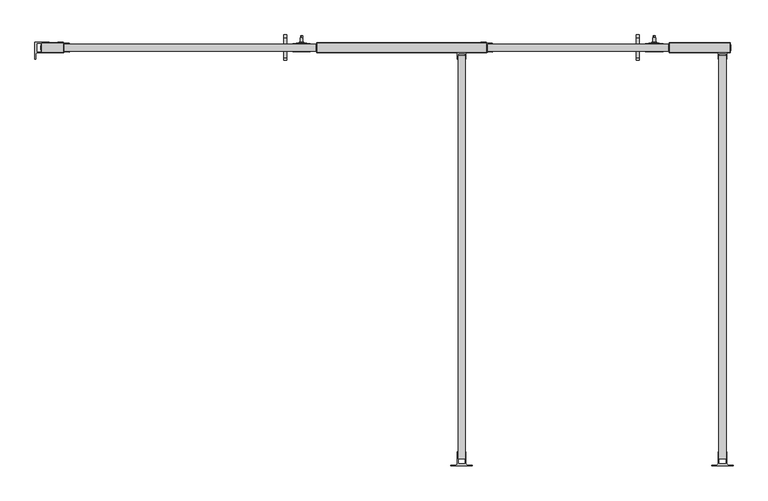
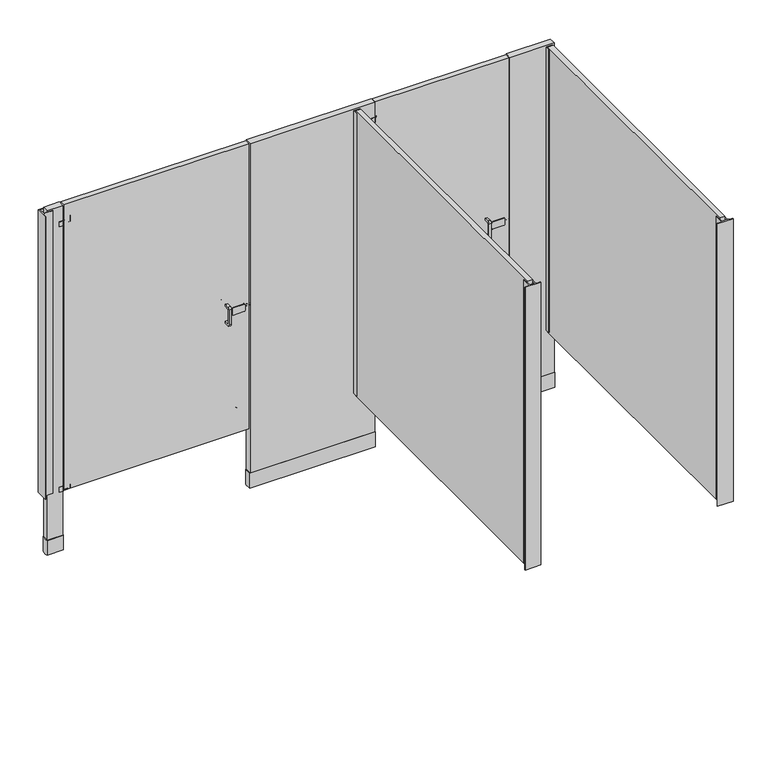
"""IFC4 building model written with IfcOpenShell, lengths in millimetres: proxy geometry, Partition-Floor_Braced-Bradley_Corp-St_Stl-ADA-N_Stalls : ADA (optional) + n Standard Stalls."""

from ifc_helpers import new_model, si_unit, point, frame, frame_2d, origin, origin_with_axes, place, context, project, spatial, polyline, circle_curve, ellipse_curve, trimmed, segment, composite_curve, outline, extrude, source, transform, mapped, element, save
from ifc_brep_helpers import plane_surface, cylinder_surface, revolved_surface, advanced_brep


def specialty_equipment_70690a28(model_context):
    return source(origin(), model_context, "Body", "SolidModel", [
        extrude(outline(composite_curve([segment(polyline([(1469.3891724, 988.06), (1492.2491724, 988.06), (1492.2491724, 977.9), (1469.3891724, 977.9)]), True, "CONTINUOUS"), segment(trimmed(circle_curve(frame_2d((1469.3891724, 975.36)), 2.54), [point((1469.3891724, 977.9))], [point((1466.8491724, 975.36))], True, "CARTESIAN"), True, "CONTINUOUS"), segment(polyline([(1466.8491724, 975.36), (1466.8491724, 904.24)]), True, "CONTINUOUS"), segment(trimmed(circle_curve(frame_2d((1469.3891724, 904.24)), 2.54), [point((1466.8491724, 904.24))], [point((1469.3891724, 901.7))], True, "CARTESIAN"), True, "CONTINUOUS"), segment(polyline([(1469.3891724, 901.7), (1492.2491724, 901.7), (1492.2491724, 891.54), (1469.3891724, 891.54)]), True, "CONTINUOUS"), segment(trimmed(circle_curve(frame_2d((1469.3891724, 901.7)), 10.16), [point((1469.3891724, 891.54))], [point((1459.2291724, 901.7))], False, "CARTESIAN"), True, "CONTINUOUS"), segment(polyline([(1459.2291724, 901.7), (1459.2291724, 977.9)]), True, "CONTINUOUS"), segment(trimmed(circle_curve(frame_2d((1469.3891724, 977.9)), 10.16), [point((1459.2291724, 977.9))], [point((1469.3891724, 988.06))], False, "CARTESIAN"), True, "CONTINUOUS")], self_intersect=False)), frame((1086.5228738, 0.0, 0.0), z_axis=(1.0, 0.0, 0.0), x_axis=(0.0, 1.0, 0.0)), (0.0, 0.0, 1.0), 11.4113578),
        extrude(outline(composite_curve([segment(trimmed(circle_curve(frame_2d((1540.51, 977.9)), 10.16), [point((1540.51, 988.06))], [point((1550.67, 977.9))], False, "CARTESIAN"), True, "CONTINUOUS"), segment(polyline([(1550.67, 977.9), (1550.67, 901.7)]), True, "CONTINUOUS"), segment(trimmed(circle_curve(frame_2d((1540.51, 901.7)), 10.16), [point((1550.67, 901.7))], [point((1540.51, 891.54))], False, "CARTESIAN"), True, "CONTINUOUS"), segment(polyline([(1540.51, 891.54), (1517.65, 891.54), (1517.65, 901.7), (1540.51, 901.7)]), True, "CONTINUOUS"), segment(trimmed(circle_curve(frame_2d((1540.51, 904.24)), 2.54), [point((1540.51, 901.7))], [point((1543.05, 904.24))], True, "CARTESIAN"), True, "CONTINUOUS"), segment(polyline([(1543.05, 904.24), (1543.05, 975.36)]), True, "CONTINUOUS"), segment(trimmed(circle_curve(frame_2d((1540.51, 975.36)), 2.54), [point((1543.05, 975.36))], [point((1540.51, 977.9))], True, "CARTESIAN"), True, "CONTINUOUS"), segment(polyline([(1540.51, 977.9), (1517.65, 977.9), (1517.65, 988.06), (1540.51, 988.06)]), True, "CONTINUOUS")], self_intersect=False)), frame((1086.5228738, 0.0, 0.0), z_axis=(1.0, 0.0, 0.0), x_axis=(0.0, 1.0, 0.0)), (0.0, 0.0, 1.0), 11.4113578),
        extrude(outline(composite_curve([segment(trimmed(circle_curve(frame_2d((406.4, 1150.9250547)), 3.4532283), [point((402.9467717, 1150.9250547))], [point((409.8532283, 1150.9250547))], False, "CARTESIAN"), True, "CONTINUOUS"), segment(trimmed(circle_curve(frame_2d((406.4, 1150.9250547)), 3.4532283), [point((409.8532283, 1150.9250547))], [point((402.9467717, 1150.9250547))], False, "CARTESIAN"), True, "CONTINUOUS")], self_intersect=False)), frame((0.0, 1540.51, 0.0), z_axis=(0.0, 1.0, 0.0), x_axis=(0.0, 0.0, 1.0)), (0.0, 0.0, 1.0), 7.62),
        advanced_brep(
        [(1150.9250547, 1517.65, 406.4), (1169.9750547, 1517.65, 406.4), (1131.8750547, 1517.65, 406.4), (1156.0050547, 1540.51, 406.4), (1150.9250547, 1540.51, 406.4), (1145.8450547, 1540.51, 406.4), (1156.0050547, 1525.27, 406.4), (1145.8450547, 1525.27, 406.4), (1161.0850547, 1520.19, 406.4), (1140.7650547, 1520.19, 406.4), (1169.9750547, 1520.19, 406.4), (1131.8750547, 1520.19, 406.4)],
        [
            (0, 1),
            (1, 2, circle_curve(frame((1150.9250547, 1517.65, 406.4), z_axis=(0.0, -1.0, 0.0), x_axis=(-1.0, 0.0, 0.0)), 19.05)),
            (2, 0),
            (2, 1, circle_curve(frame((1150.9250547, 1517.65, 406.4), z_axis=(0.0, -1.0, 0.0), x_axis=(-1.0, 0.0, 0.0)), 19.05)),
            (3, 4),
            (4, 5),
            (5, 3, circle_curve(frame((1150.9250547, 1540.51, 406.4), z_axis=(0.0, 1.0, 0.0), x_axis=(-1.0, 0.0, 0.0)), 5.08)),
            (3, 5, circle_curve(frame((1150.9250547, 1540.51, 406.4), z_axis=(0.0, 1.0, 0.0), x_axis=(-1.0, 0.0, 0.0)), 5.08)),
            (6, 3),
            (5, 7),
            (7, 6, circle_curve(frame((1150.9250547, 1525.27, 406.4), z_axis=(0.0, 1.0, 0.0), x_axis=(-1.0, 0.0, 0.0)), 5.08)),
            (6, 7, circle_curve(frame((1150.9250547, 1525.27, 406.4), z_axis=(0.0, 1.0, 0.0), x_axis=(-1.0, 0.0, 0.0)), 5.08)),
            (8, 6, circle_curve(frame((1156.0050547, 1520.19, 406.4), z_axis=(0.0, 0.0, 1.0), x_axis=(0.0, 1.0, 0.0)), 5.08)),
            (7, 9, circle_curve(frame((1145.8450547, 1520.19, 406.4), z_axis=(0.0, 0.0, 1.0), x_axis=(0.0, 1.0, 0.0)), 5.08)),
            (9, 8, circle_curve(frame((1150.9250547, 1520.19, 406.4), z_axis=(0.0, 1.0, 0.0), x_axis=(-1.0, 0.0, 0.0)), 10.16)),
            (8, 9, circle_curve(frame((1150.9250547, 1520.19, 406.4), z_axis=(0.0, 1.0, 0.0), x_axis=(-1.0, 0.0, 0.0)), 10.16)),
            (10, 8),
            (9, 11),
            (11, 10, circle_curve(frame((1150.9250547, 1520.19, 406.4), z_axis=(0.0, 1.0, 0.0), x_axis=(-1.0, 0.0, 0.0)), 19.05)),
            (10, 11, circle_curve(frame((1150.9250547, 1520.19, 406.4), z_axis=(0.0, 1.0, 0.0), x_axis=(-1.0, 0.0, 0.0)), 19.05)),
            (1, 10),
            (11, 2),
        ],
        [
            plane_surface(frame((1150.9250547, 1517.65, 406.4), z_axis=(0.0, -1.0, 0.0), x_axis=(-1.0, 0.0, 0.0))),
            plane_surface(frame((1150.9250547, 1540.51, 406.4), z_axis=(0.0, 1.0, 0.0), x_axis=(-1.0, 0.0, 0.0))),
            cylinder_surface(frame((1150.9250547, 1561.6297247, 406.4), z_axis=(0.0, -1.0, 0.0), x_axis=(-1.0, 0.0, 0.0)), 5.08),
            revolved_surface(trimmed(ellipse_curve(frame((1145.8450547, 1520.19, 406.4), z_axis=(0.0, 0.0, 1.0), x_axis=(0.0, 1.0, 0.0)), 5.08, 5.08), [point((1145.8450547, 1525.27, 406.4))], [point((1140.7650547, 1520.19, 406.4))], True, "CARTESIAN"), (1150.9250547, 1561.6297247, 406.4), (0.0, -1.0, 0.0)),
            plane_surface(frame((1150.9250547, 1520.19, 406.4), z_axis=(0.0, 1.0, 0.0), x_axis=(-1.0, 0.0, 0.0))),
            cylinder_surface(frame((1150.9250547, 1561.6297247, 406.4), z_axis=(0.0, -1.0, 0.0), x_axis=(-1.0, 0.0, 0.0)), 19.05),
        ],
        [
            (0, [[1, 2, 3]]),
            (0, [[-3, 4, -1]]),
            (1, [[5, 6, 7]]),
            (1, [[-6, -5, 8]]),
            (2, [[9, -7, 10, 11]]),
            (2, [[-10, -8, -9, 12]]),
            (3, [[13, -11, 14, 15]]),
            (3, [[-14, -12, -13, 16]]),
            (4, [[17, -15, 18, 19]]),
            (4, [[-18, -16, -17, 20]]),
            (5, [[21, -19, 22, -2]]),
            (5, [[-22, -20, -21, -4]]),
        ],
    ),
        advanced_brep(
        [(1195.3750547, 1499.87, 939.8), (1212.8502547, 1499.87, 939.8), (1212.8502547, 1510.03, 939.8), (1195.3750547, 1510.03, 939.8), (1195.3750547, 1504.95, 939.8), (1212.8502547, 1504.95, 939.8)],
        [
            (0, 1),
            (1, 2, circle_curve(frame((1212.8502547, 1504.95, 939.8), z_axis=(-1.0, 0.0, 0.0), x_axis=(0.0, 1.0, 0.0)), 5.08)),
            (2, 3),
            (3, 0, circle_curve(frame((1195.3750547, 1504.95, 939.8), z_axis=(1.0, 0.0, 0.0), x_axis=(0.0, 1.0, 0.0)), 5.08)),
            (2, 1, circle_curve(frame((1212.8502547, 1504.95, 939.8), z_axis=(-1.0, 0.0, 0.0), x_axis=(0.0, 1.0, 0.0)), 5.08)),
            (0, 3, circle_curve(frame((1195.3750547, 1504.95, 939.8), z_axis=(1.0, 0.0, 0.0), x_axis=(0.0, 1.0, 0.0)), 5.08)),
            (4, 0),
            (3, 4),
            (1, 5),
            (5, 2),
        ],
        [
            cylinder_surface(frame((1212.8502547, 1504.95, 939.8), z_axis=(-1.0, 0.0, 0.0), x_axis=(0.0, 1.0, 0.0)), 5.08),
            plane_surface(frame((1195.3750547, 1504.95, 939.8), z_axis=(-1.0, 0.0, 0.0), x_axis=(0.0, 1.0, 0.0))),
            plane_surface(frame((1212.8502547, 1504.95, 939.8), z_axis=(1.0, 0.0, 0.0), x_axis=(0.0, 1.0, 0.0))),
        ],
        [
            (0, [[1, 2, 3, 4]]),
            (0, [[-3, 5, -1, 6]]),
            (1, [[7, -4, 8]]),
            (1, [[-8, -6, -7]]),
            (2, [[9, 10, -2]]),
            (2, [[-10, -9, -5]]),
        ],
    ),
        extrude(outline(composite_curve([segment(trimmed(circle_curve(frame_2d((926.0058992, 1124.4309539)), 5.2558992), [point((926.0058992, 1119.1750547))], [point((920.75, 1124.4309539))], False, "CARTESIAN"), True, "CONTINUOUS"), segment(polyline([(920.75, 1124.4309539), (920.75, 1177.4191555)]), True, "CONTINUOUS"), segment(trimmed(circle_curve(frame_2d((926.0058992, 1177.4191555)), 5.2558992), [point((920.75, 1177.4191555))], [point((926.0058992, 1182.6750547))], False, "CARTESIAN"), True, "CONTINUOUS"), segment(polyline([(926.0058992, 1182.6750547), (953.5941008, 1182.6750547)]), True, "CONTINUOUS"), segment(trimmed(circle_curve(frame_2d((953.5941008, 1177.4191555)), 5.2558992), [point((953.5941008, 1182.6750547))], [point((958.85, 1177.4191555))], False, "CARTESIAN"), True, "CONTINUOUS"), segment(polyline([(958.85, 1177.4191555), (958.85, 1124.4309539)]), True, "CONTINUOUS"), segment(trimmed(circle_curve(frame_2d((953.5941008, 1124.4309539)), 5.2558992), [point((958.85, 1124.4309539))], [point((953.5941008, 1119.1750547))], False, "CARTESIAN"), True, "CONTINUOUS"), segment(polyline([(953.5941008, 1119.1750547), (926.0058992, 1119.1750547)]), True, "CONTINUOUS")], self_intersect=False)), frame((0.0, 1490.345, 0.0), z_axis=(0.0, 1.0, 0.0), x_axis=(0.0, 0.0, 1.0)), (0.0, 0.0, 1.0), 29.21),
        extrude(outline(composite_curve([segment(polyline([(1469.3891724, 988.06), (1492.2491724, 988.06), (1492.2491724, 977.9), (1469.3891724, 977.9)]), True, "CONTINUOUS"), segment(trimmed(circle_curve(frame_2d((1469.3891724, 975.36)), 2.54), [point((1469.3891724, 977.9))], [point((1466.8491724, 975.36))], True, "CARTESIAN"), True, "CONTINUOUS"), segment(polyline([(1466.8491724, 975.36), (1466.8491724, 904.24)]), True, "CONTINUOUS"), segment(trimmed(circle_curve(frame_2d((1469.3891724, 904.24)), 2.54), [point((1466.8491724, 904.24))], [point((1469.3891724, 901.7))], True, "CARTESIAN"), True, "CONTINUOUS"), segment(polyline([(1469.3891724, 901.7), (1492.2491724, 901.7), (1492.2491724, 891.54), (1469.3891724, 891.54)]), True, "CONTINUOUS"), segment(trimmed(circle_curve(frame_2d((1469.3891724, 901.7)), 10.16), [point((1469.3891724, 891.54))], [point((1459.2291724, 901.7))], False, "CARTESIAN"), True, "CONTINUOUS"), segment(polyline([(1459.2291724, 901.7), (1459.2291724, 977.9)]), True, "CONTINUOUS"), segment(trimmed(circle_curve(frame_2d((1469.3891724, 977.9)), 10.16), [point((1459.2291724, 977.9))], [point((1469.3891724, 988.06))], False, "CARTESIAN"), True, "CONTINUOUS")], self_intersect=False)), frame((2356.5228738, 0.0, 0.0), z_axis=(1.0, 0.0, 0.0), x_axis=(0.0, 1.0, 0.0)), (0.0, 0.0, 1.0), 11.4113578),
        extrude(outline(composite_curve([segment(trimmed(circle_curve(frame_2d((1540.51, 977.9)), 10.16), [point((1540.51, 988.06))], [point((1550.67, 977.9))], False, "CARTESIAN"), True, "CONTINUOUS"), segment(polyline([(1550.67, 977.9), (1550.67, 901.7)]), True, "CONTINUOUS"), segment(trimmed(circle_curve(frame_2d((1540.51, 901.7)), 10.16), [point((1550.67, 901.7))], [point((1540.51, 891.54))], False, "CARTESIAN"), True, "CONTINUOUS"), segment(polyline([(1540.51, 891.54), (1517.65, 891.54), (1517.65, 901.7), (1540.51, 901.7)]), True, "CONTINUOUS"), segment(trimmed(circle_curve(frame_2d((1540.51, 904.24)), 2.54), [point((1540.51, 901.7))], [point((1543.05, 904.24))], True, "CARTESIAN"), True, "CONTINUOUS"), segment(polyline([(1543.05, 904.24), (1543.05, 975.36)]), True, "CONTINUOUS"), segment(trimmed(circle_curve(frame_2d((1540.51, 975.36)), 2.54), [point((1543.05, 975.36))], [point((1540.51, 977.9))], True, "CARTESIAN"), True, "CONTINUOUS"), segment(polyline([(1540.51, 977.9), (1517.65, 977.9), (1517.65, 988.06), (1540.51, 988.06)]), True, "CONTINUOUS")], self_intersect=False)), frame((2356.5228738, 0.0, 0.0), z_axis=(1.0, 0.0, 0.0), x_axis=(0.0, 1.0, 0.0)), (0.0, 0.0, 1.0), 11.4113578),
        extrude(outline(composite_curve([segment(trimmed(circle_curve(frame_2d((406.4, 2420.9250547)), 3.4532283), [point((402.9467717, 2420.9250547))], [point((409.8532283, 2420.9250547))], False, "CARTESIAN"), True, "CONTINUOUS"), segment(trimmed(circle_curve(frame_2d((406.4, 2420.9250547)), 3.4532283), [point((409.8532283, 2420.9250547))], [point((402.9467717, 2420.9250547))], False, "CARTESIAN"), True, "CONTINUOUS")], self_intersect=False)), frame((0.0, 1540.51, 0.0), z_axis=(0.0, 1.0, 0.0), x_axis=(0.0, 0.0, 1.0)), (0.0, 0.0, 1.0), 7.62),
        advanced_brep(
        [(2420.9250547, 1517.65, 406.4), (2439.9750547, 1517.65, 406.4), (2401.8750547, 1517.65, 406.4), (2426.0050547, 1540.51, 406.4), (2420.9250547, 1540.51, 406.4), (2415.8450547, 1540.51, 406.4), (2426.0050547, 1525.27, 406.4), (2415.8450547, 1525.27, 406.4), (2431.0850547, 1520.19, 406.4), (2410.7650547, 1520.19, 406.4), (2439.9750547, 1520.19, 406.4), (2401.8750547, 1520.19, 406.4)],
        [
            (0, 1),
            (1, 2, circle_curve(frame((2420.9250547, 1517.65, 406.4), z_axis=(0.0, -1.0, 0.0), x_axis=(-1.0, 0.0, 0.0)), 19.05)),
            (2, 0),
            (2, 1, circle_curve(frame((2420.9250547, 1517.65, 406.4), z_axis=(0.0, -1.0, 0.0), x_axis=(-1.0, 0.0, 0.0)), 19.05)),
            (3, 4),
            (4, 5),
            (5, 3, circle_curve(frame((2420.9250547, 1540.51, 406.4), z_axis=(0.0, 1.0, 0.0), x_axis=(-1.0, 0.0, 0.0)), 5.08)),
            (3, 5, circle_curve(frame((2420.9250547, 1540.51, 406.4), z_axis=(0.0, 1.0, 0.0), x_axis=(-1.0, 0.0, 0.0)), 5.08)),
            (6, 3),
            (5, 7),
            (7, 6, circle_curve(frame((2420.9250547, 1525.27, 406.4), z_axis=(0.0, 1.0, 0.0), x_axis=(-1.0, 0.0, 0.0)), 5.08)),
            (6, 7, circle_curve(frame((2420.9250547, 1525.27, 406.4), z_axis=(0.0, 1.0, 0.0), x_axis=(-1.0, 0.0, 0.0)), 5.08)),
            (8, 6, circle_curve(frame((2426.0050547, 1520.19, 406.4), z_axis=(0.0, 0.0, 1.0), x_axis=(0.0, 1.0, 0.0)), 5.08)),
            (7, 9, circle_curve(frame((2415.8450547, 1520.19, 406.4), z_axis=(0.0, 0.0, 1.0), x_axis=(0.0, 1.0, 0.0)), 5.08)),
            (9, 8, circle_curve(frame((2420.9250547, 1520.19, 406.4), z_axis=(0.0, 1.0, 0.0), x_axis=(-1.0, 0.0, 0.0)), 10.16)),
            (8, 9, circle_curve(frame((2420.9250547, 1520.19, 406.4), z_axis=(0.0, 1.0, 0.0), x_axis=(-1.0, 0.0, 0.0)), 10.16)),
            (10, 8),
            (9, 11),
            (11, 10, circle_curve(frame((2420.9250547, 1520.19, 406.4), z_axis=(0.0, 1.0, 0.0), x_axis=(-1.0, 0.0, 0.0)), 19.05)),
            (10, 11, circle_curve(frame((2420.9250547, 1520.19, 406.4), z_axis=(0.0, 1.0, 0.0), x_axis=(-1.0, 0.0, 0.0)), 19.05)),
            (1, 10),
            (11, 2),
        ],
        [
            plane_surface(frame((2420.9250547, 1517.65, 406.4), z_axis=(0.0, -1.0, 0.0), x_axis=(-1.0, 0.0, 0.0))),
            plane_surface(frame((2420.9250547, 1540.51, 406.4), z_axis=(0.0, 1.0, 0.0), x_axis=(-1.0, 0.0, 0.0))),
            cylinder_surface(frame((2420.9250547, 1561.6297247, 406.4), z_axis=(0.0, -1.0, 0.0), x_axis=(-1.0, 0.0, 0.0)), 5.08),
            revolved_surface(trimmed(ellipse_curve(frame((2415.8450547, 1520.19, 406.4), z_axis=(0.0, 0.0, 1.0), x_axis=(0.0, 1.0, 0.0)), 5.08, 5.08), [point((2415.8450547, 1525.27, 406.4))], [point((2410.7650547, 1520.19, 406.4))], True, "CARTESIAN"), (2420.9250547, 1561.6297247, 406.4), (0.0, -1.0, 0.0)),
            plane_surface(frame((2420.9250547, 1520.19, 406.4), z_axis=(0.0, 1.0, 0.0), x_axis=(-1.0, 0.0, 0.0))),
            cylinder_surface(frame((2420.9250547, 1561.6297247, 406.4), z_axis=(0.0, -1.0, 0.0), x_axis=(-1.0, 0.0, 0.0)), 19.05),
        ],
        [
            (0, [[1, 2, 3]]),
            (0, [[-3, 4, -1]]),
            (1, [[5, 6, 7]]),
            (1, [[-6, -5, 8]]),
            (2, [[9, -7, 10, 11]]),
            (2, [[-10, -8, -9, 12]]),
            (3, [[13, -11, 14, 15]]),
            (3, [[-14, -12, -13, 16]]),
            (4, [[17, -15, 18, 19]]),
            (4, [[-18, -16, -17, 20]]),
            (5, [[21, -19, 22, -2]]),
            (5, [[-22, -20, -21, -4]]),
        ],
    ),
        advanced_brep(
        [(2465.3750547, 1499.87, 939.8), (2482.8502547, 1499.87, 939.8), (2482.8502547, 1510.03, 939.8), (2465.3750547, 1510.03, 939.8), (2465.3750547, 1504.95, 939.8), (2482.8502547, 1504.95, 939.8)],
        [
            (0, 1),
            (1, 2, circle_curve(frame((2482.8502547, 1504.95, 939.8), z_axis=(-1.0, 0.0, 0.0), x_axis=(0.0, 1.0, 0.0)), 5.08)),
            (2, 3),
            (3, 0, circle_curve(frame((2465.3750547, 1504.95, 939.8), z_axis=(1.0, 0.0, 0.0), x_axis=(0.0, 1.0, 0.0)), 5.08)),
            (2, 1, circle_curve(frame((2482.8502547, 1504.95, 939.8), z_axis=(-1.0, 0.0, 0.0), x_axis=(0.0, 1.0, 0.0)), 5.08)),
            (0, 3, circle_curve(frame((2465.3750547, 1504.95, 939.8), z_axis=(1.0, 0.0, 0.0), x_axis=(0.0, 1.0, 0.0)), 5.08)),
            (4, 0),
            (3, 4),
            (1, 5),
            (5, 2),
        ],
        [
            cylinder_surface(frame((2482.8502547, 1504.95, 939.8), z_axis=(-1.0, 0.0, 0.0), x_axis=(0.0, 1.0, 0.0)), 5.08),
            plane_surface(frame((2465.3750547, 1504.95, 939.8), z_axis=(-1.0, 0.0, 0.0), x_axis=(0.0, 1.0, 0.0))),
            plane_surface(frame((2482.8502547, 1504.95, 939.8), z_axis=(1.0, 0.0, 0.0), x_axis=(0.0, 1.0, 0.0))),
        ],
        [
            (0, [[1, 2, 3, 4]]),
            (0, [[-3, 5, -1, 6]]),
            (1, [[7, -4, 8]]),
            (1, [[-8, -6, -7]]),
            (2, [[9, 10, -2]]),
            (2, [[-10, -9, -5]]),
        ],
    ),
        extrude(outline(composite_curve([segment(trimmed(circle_curve(frame_2d((926.0058992, 2394.4309539)), 5.2558992), [point((926.0058992, 2389.1750547))], [point((920.75, 2394.4309539))], False, "CARTESIAN"), True, "CONTINUOUS"), segment(polyline([(920.75, 2394.4309539), (920.75, 2447.4191555)]), True, "CONTINUOUS"), segment(trimmed(circle_curve(frame_2d((926.0058992, 2447.4191555)), 5.2558992), [point((920.75, 2447.4191555))], [point((926.0058992, 2452.6750547))], False, "CARTESIAN"), True, "CONTINUOUS"), segment(polyline([(926.0058992, 2452.6750547), (953.5941008, 2452.6750547)]), True, "CONTINUOUS"), segment(trimmed(circle_curve(frame_2d((953.5941008, 2447.4191555)), 5.2558992), [point((953.5941008, 2452.6750547))], [point((958.85, 2447.4191555))], False, "CARTESIAN"), True, "CONTINUOUS"), segment(polyline([(958.85, 2447.4191555), (958.85, 2394.4309539)]), True, "CONTINUOUS"), segment(trimmed(circle_curve(frame_2d((953.5941008, 2394.4309539)), 5.2558992), [point((958.85, 2394.4309539))], [point((953.5941008, 2389.1750547))], False, "CARTESIAN"), True, "CONTINUOUS"), segment(polyline([(953.5941008, 2389.1750547), (926.0058992, 2389.1750547)]), True, "CONTINUOUS")], self_intersect=False)), frame((0.0, 1490.345, 0.0), z_axis=(0.0, 1.0, 0.0), x_axis=(0.0, 0.0, 1.0)), (0.0, 0.0, 1.0), 29.21),
        extrude(outline(composite_curve([segment(trimmed(circle_curve(frame_2d((1825.9554547, 1504.95)), 2.54), [point((1825.9554547, 1507.49))], [point((1825.9554547, 1502.41))], False, "CARTESIAN"), True, "CONTINUOUS"), segment(trimmed(circle_curve(frame_2d((1825.9554547, 1504.95)), 2.54), [point((1825.9554547, 1502.41))], [point((1825.9554547, 1507.49))], False, "CARTESIAN"), True, "CONTINUOUS")], self_intersect=False)), frame((0.0, 0.0, 304.8), z_axis=(0.0, 0.0, 1.0), x_axis=(1.0, 0.0, 0.0)), (0.0, 0.0, 1.0), 25.4),
        extrude(outline(composite_curve([segment(polyline([(1816.1002547, 1489.71), (1816.1002547, 1520.19), (1837.6902547, 1520.825), (1847.8502547, 1512.57)]), True, "CONTINUOUS"), segment(trimmed(circle_curve(frame_2d((1844.0402547, 1504.95)), 8.519419), [point((1847.8502547, 1512.57))], [point((1847.8502547, 1497.33))], False, "CARTESIAN"), True, "CONTINUOUS"), segment(polyline([(1847.8502547, 1497.33), (1837.6902547, 1489.075), (1816.1002547, 1489.71)]), True, "CONTINUOUS")], self_intersect=False)), frame((0.0, 0.0, 304.8), z_axis=(0.0, 0.0, 1.0), x_axis=(1.0, 0.0, 0.0)), (0.0, 0.0, 1.0), 3.81),
        extrude(outline(composite_curve([segment(polyline([(1797.0502547, 1486.535), (1797.0502547, 1523.365), (1816.1002547, 1523.365)]), True, "CONTINUOUS"), segment(trimmed(circle_curve(frame_2d((1816.1002547, 1520.825)), 2.54), [point((1816.1002547, 1523.365))], [point((1818.6402547, 1520.825))], False, "CARTESIAN"), True, "CONTINUOUS"), segment(trimmed(circle_curve(frame_2d((1710.8397496, 1504.95)), 108.9631338), [point((1818.6402547, 1520.825))], [point((1818.6402547, 1489.075))], False, "CARTESIAN"), True, "CONTINUOUS"), segment(trimmed(circle_curve(frame_2d((1816.1002547, 1489.075)), 2.54), [point((1818.6402547, 1489.075))], [point((1816.1002547, 1486.535))], False, "CARTESIAN"), True, "CONTINUOUS"), segment(polyline([(1816.1002547, 1486.535), (1797.0502547, 1486.535)]), True, "CONTINUOUS")], self_intersect=False)), frame((0.0, 0.0, 304.8), z_axis=(0.0, 0.0, 1.0), x_axis=(1.0, 0.0, 0.0)), (0.0, 0.0, 1.0), 25.4),
        extrude(outline(composite_curve([segment(trimmed(circle_curve(frame_2d((1825.9554547, 1504.95)), 2.54), [point((1825.9554547, 1507.49))], [point((1825.9554547, 1502.41))], False, "CARTESIAN"), True, "CONTINUOUS"), segment(trimmed(circle_curve(frame_2d((1825.9554547, 1504.95)), 2.54), [point((1825.9554547, 1502.41))], [point((1825.9554547, 1507.49))], False, "CARTESIAN"), True, "CONTINUOUS")], self_intersect=False)), frame((0.0, 0.0, 1676.4), z_axis=(0.0, 0.0, 1.0), x_axis=(1.0, 0.0, 0.0)), (0.0, 0.0, 1.0), 25.4),
        extrude(outline(composite_curve([segment(polyline([(1820.8754547, 1520.825), (1831.0354547, 1512.57)]), True, "CONTINUOUS"), segment(trimmed(circle_curve(frame_2d((1827.2254547, 1504.95)), 8.519419), [point((1831.0354547, 1512.57))], [point((1831.0354547, 1497.33))], False, "CARTESIAN"), True, "CONTINUOUS"), segment(polyline([(1831.0354547, 1497.33), (1820.8754547, 1489.075), (1816.1002547, 1489.71), (1816.1002547, 1520.19), (1820.8754547, 1520.825)]), True, "CONTINUOUS")], self_intersect=False)), frame((0.0, 0.0, 1697.99), z_axis=(0.0, 0.0, 1.0), x_axis=(1.0, 0.0, 0.0)), (0.0, 0.0, 1.0), 3.81),
        extrude(outline(composite_curve([segment(polyline([(1797.0502547, 1486.535), (1797.0502547, 1523.365), (1816.1002547, 1523.365)]), True, "CONTINUOUS"), segment(trimmed(circle_curve(frame_2d((1816.1002547, 1520.825)), 2.54), [point((1816.1002547, 1523.365))], [point((1818.6402547, 1520.825))], False, "CARTESIAN"), True, "CONTINUOUS"), segment(trimmed(circle_curve(frame_2d((1710.8397496, 1504.95)), 108.9631338), [point((1818.6402547, 1520.825))], [point((1818.6402547, 1489.075))], False, "CARTESIAN"), True, "CONTINUOUS"), segment(trimmed(circle_curve(frame_2d((1816.1002547, 1489.075)), 2.54), [point((1818.6402547, 1489.075))], [point((1816.1002547, 1486.535))], False, "CARTESIAN"), True, "CONTINUOUS"), segment(polyline([(1816.1002547, 1486.535), (1797.0502547, 1486.535)]), True, "CONTINUOUS")], self_intersect=False)), frame((0.0, 0.0, 1676.4), z_axis=(0.0, 0.0, 1.0), x_axis=(1.0, 0.0, 0.0)), (0.0, 0.0, 1.0), 25.4),
        extrude(outline(polyline([(2651.7602547, 1489.075), (2682.2402547, 1489.075), (2682.2402547, 1463.675), (2679.7002547, 1463.675), (2679.7002547, 1482.1271812), (2654.3002547, 1482.1271812), (2654.3002547, 1463.675), (2651.7602547, 1463.675), (2651.7602547, 1489.075)])), frame((0.0, 0.0, 311.15), z_axis=(0.0, 0.0, 1.0), x_axis=(1.0, 0.0, 0.0)), (0.0, 0.0, 1.0), 1460.5),
        extrude(outline(composite_curve([segment(polyline([(2705.1002547, -3.175), (2628.9002547, -3.175), (2628.9002547, -0.635), (2645.4102547, -0.635)]), True, "CONTINUOUS"), segment(trimmed(circle_curve(frame_2d((2645.4102547, 5.715)), 6.35), [point((2645.4102547, -0.635))], [point((2651.7602547, 5.715))], True, "CARTESIAN"), True, "CONTINUOUS"), segment(polyline([(2651.7602547, 5.715), (2651.7602547, 47.625), (2654.3002547, 47.625), (2654.3002547, 3.7728188), (2679.7002547, 3.7728188), (2679.7002547, 47.625), (2682.2402547, 47.625), (2682.2402547, 5.715)]), True, "CONTINUOUS"), segment(trimmed(circle_curve(frame_2d((2688.5902547, 5.715)), 6.35), [point((2682.2402547, 5.715))], [point((2688.5902547, -0.635))], True, "CARTESIAN"), True, "CONTINUOUS"), segment(polyline([(2688.5902547, -0.635), (2705.1002547, -0.635), (2705.1002547, -3.175)]), True, "CONTINUOUS")], self_intersect=False)), frame((0.0, 0.0, 311.15), z_axis=(0.0, 0.0, 1.0), x_axis=(1.0, 0.0, 0.0)), (0.0, 0.0, 1.0), 1460.5),
        extrude(outline(composite_curve([segment(trimmed(circle_curve(frame_2d((301.9554547, 1504.95)), 2.54), [point((301.9554547, 1507.49))], [point((301.9554547, 1502.41))], False, "CARTESIAN"), True, "CONTINUOUS"), segment(trimmed(circle_curve(frame_2d((301.9554547, 1504.95)), 2.54), [point((301.9554547, 1502.41))], [point((301.9554547, 1507.49))], False, "CARTESIAN"), True, "CONTINUOUS")], self_intersect=False)), frame((0.0, 0.0, 304.8), z_axis=(0.0, 0.0, 1.0), x_axis=(1.0, 0.0, 0.0)), (0.0, 0.0, 1.0), 25.4),
        extrude(outline(composite_curve([segment(polyline([(292.1002547, 1489.71), (292.1002547, 1520.19), (313.6902547, 1520.825), (323.8502547, 1512.57)]), True, "CONTINUOUS"), segment(trimmed(circle_curve(frame_2d((320.0402547, 1504.95)), 8.519419), [point((323.8502547, 1512.57))], [point((323.8502547, 1497.33))], False, "CARTESIAN"), True, "CONTINUOUS"), segment(polyline([(323.8502547, 1497.33), (313.6902547, 1489.075), (292.1002547, 1489.71)]), True, "CONTINUOUS")], self_intersect=False)), frame((0.0, 0.0, 304.8), z_axis=(0.0, 0.0, 1.0), x_axis=(1.0, 0.0, 0.0)), (0.0, 0.0, 1.0), 3.81),
        extrude(outline(composite_curve([segment(polyline([(273.0502547, 1486.535), (273.0502547, 1523.365), (292.1002547, 1523.365)]), True, "CONTINUOUS"), segment(trimmed(circle_curve(frame_2d((292.1002547, 1520.825)), 2.54), [point((292.1002547, 1523.365))], [point((294.6402547, 1520.825))], False, "CARTESIAN"), True, "CONTINUOUS"), segment(trimmed(circle_curve(frame_2d((186.8397496, 1504.95)), 108.9631338), [point((294.6402547, 1520.825))], [point((294.6402547, 1489.075))], False, "CARTESIAN"), True, "CONTINUOUS"), segment(trimmed(circle_curve(frame_2d((292.1002547, 1489.075)), 2.54), [point((294.6402547, 1489.075))], [point((292.1002547, 1486.535))], False, "CARTESIAN"), True, "CONTINUOUS"), segment(polyline([(292.1002547, 1486.535), (273.0502547, 1486.535)]), True, "CONTINUOUS")], self_intersect=False)), frame((0.0, 0.0, 304.8), z_axis=(0.0, 0.0, 1.0), x_axis=(1.0, 0.0, 0.0)), (0.0, 0.0, 1.0), 25.4),
        extrude(outline(composite_curve([segment(trimmed(circle_curve(frame_2d((301.9554547, 1504.95)), 2.54), [point((301.9554547, 1507.49))], [point((301.9554547, 1502.41))], False, "CARTESIAN"), True, "CONTINUOUS"), segment(trimmed(circle_curve(frame_2d((301.9554547, 1504.95)), 2.54), [point((301.9554547, 1502.41))], [point((301.9554547, 1507.49))], False, "CARTESIAN"), True, "CONTINUOUS")], self_intersect=False)), frame((0.0, 0.0, 1676.4), z_axis=(0.0, 0.0, 1.0), x_axis=(1.0, 0.0, 0.0)), (0.0, 0.0, 1.0), 25.4),
        extrude(outline(composite_curve([segment(polyline([(296.8754547, 1520.825), (307.0354547, 1512.57)]), True, "CONTINUOUS"), segment(trimmed(circle_curve(frame_2d((303.2254547, 1504.95)), 8.519419), [point((307.0354547, 1512.57))], [point((307.0354547, 1497.33))], False, "CARTESIAN"), True, "CONTINUOUS"), segment(polyline([(307.0354547, 1497.33), (296.8754547, 1489.075), (292.1002547, 1489.71), (292.1002547, 1520.19), (296.8754547, 1520.825)]), True, "CONTINUOUS")], self_intersect=False)), frame((0.0, 0.0, 1697.99), z_axis=(0.0, 0.0, 1.0), x_axis=(1.0, 0.0, 0.0)), (0.0, 0.0, 1.0), 3.81),
        extrude(outline(composite_curve([segment(polyline([(273.0502547, 1486.535), (273.0502547, 1523.365), (292.1002547, 1523.365)]), True, "CONTINUOUS"), segment(trimmed(circle_curve(frame_2d((292.1002547, 1520.825)), 2.54), [point((292.1002547, 1523.365))], [point((294.6402547, 1520.825))], False, "CARTESIAN"), True, "CONTINUOUS"), segment(trimmed(circle_curve(frame_2d((186.8397496, 1504.95)), 108.9631338), [point((294.6402547, 1520.825))], [point((294.6402547, 1489.075))], False, "CARTESIAN"), True, "CONTINUOUS"), segment(trimmed(circle_curve(frame_2d((292.1002547, 1489.075)), 2.54), [point((294.6402547, 1489.075))], [point((292.1002547, 1486.535))], False, "CARTESIAN"), True, "CONTINUOUS"), segment(polyline([(292.1002547, 1486.535), (273.0502547, 1486.535)]), True, "CONTINUOUS")], self_intersect=False)), frame((0.0, 0.0, 1676.4), z_axis=(0.0, 0.0, 1.0), x_axis=(1.0, 0.0, 0.0)), (0.0, 0.0, 1.0), 25.4),
        extrude(outline(composite_curve([segment(polyline([(190.5002547, 1463.675), (190.5002547, 1523.365), (241.3002547, 1523.365), (241.3002547, 1520.825), (197.4480735, 1520.825), (197.4480735, 1489.075), (241.3002547, 1489.075), (241.3002547, 1486.535), (199.3902547, 1486.535)]), True, "CONTINUOUS"), segment(trimmed(circle_curve(frame_2d((199.3902547, 1480.185)), 6.35), [point((199.3902547, 1486.535))], [point((193.0402547, 1480.185))], True, "CARTESIAN"), True, "CONTINUOUS"), segment(polyline([(193.0402547, 1480.185), (193.0402547, 1463.675), (190.5002547, 1463.675)]), True, "CONTINUOUS")], self_intersect=False)), frame((0.0, 0.0, 311.15), z_axis=(0.0, 0.0, 1.0), x_axis=(1.0, 0.0, 0.0)), (0.0, 0.0, 1.0), 1460.5),
        extrude(outline(polyline([(1711.9602547, 1489.075), (1742.4402547, 1489.075), (1742.4402547, 1463.675), (1739.9002547, 1463.675), (1739.9002547, 1482.1271812), (1714.5002547, 1482.1271812), (1714.5002547, 1463.675), (1711.9602547, 1463.675), (1711.9602547, 1489.075)])), frame((0.0, 0.0, 311.15), z_axis=(0.0, 0.0, 1.0), x_axis=(1.0, 0.0, 0.0)), (0.0, 0.0, 1.0), 1460.5),
        extrude(outline(composite_curve([segment(polyline([(1765.3002547, -3.175), (1689.1002547, -3.175), (1689.1002547, -0.635), (1705.6102547, -0.635)]), True, "CONTINUOUS"), segment(trimmed(circle_curve(frame_2d((1705.6102547, 5.715)), 6.35), [point((1705.6102547, -0.635))], [point((1711.9602547, 5.715))], True, "CARTESIAN"), True, "CONTINUOUS"), segment(polyline([(1711.9602547, 5.715), (1711.9602547, 47.625), (1714.5002547, 47.625), (1714.5002547, 3.7728188), (1739.9002547, 3.7728188), (1739.9002547, 47.625), (1742.4402547, 47.625), (1742.4402547, 5.715)]), True, "CONTINUOUS"), segment(trimmed(circle_curve(frame_2d((1748.7902547, 5.715)), 6.35), [point((1742.4402547, 5.715))], [point((1748.7902547, -0.635))], True, "CARTESIAN"), True, "CONTINUOUS"), segment(polyline([(1748.7902547, -0.635), (1765.3002547, -0.635), (1765.3002547, -3.175)]), True, "CONTINUOUS")], self_intersect=False)), frame((0.0, 0.0, 311.15), z_axis=(0.0, 0.0, 1.0), x_axis=(1.0, 0.0, 0.0)), (0.0, 0.0, 1.0), 1460.5),
        extrude(outline(composite_curve([segment(trimmed(circle_curve(frame_2d((270.1017864, 1504.95)), 58.4581471), [point((214.3127547, 1487.4875))], [point((214.3127547, 1522.4125))], False, "CARTESIAN"), True, "CONTINUOUS"), segment(polyline([(214.3127547, 1522.4125), (293.6891337, 1522.4125)]), True, "CONTINUOUS"), segment(trimmed(circle_curve(frame_2d((237.900102, 1504.95)), 58.4581471), [point((293.6891337, 1522.4125))], [point((293.6891337, 1487.4875))], False, "CARTESIAN"), True, "CONTINUOUS"), segment(polyline([(293.6891337, 1487.4875), (214.3127547, 1487.4875)]), True, "CONTINUOUS")], self_intersect=False)), origin_with_axes(), (0.0, 0.0, 1.0), 76.2),
        extrude(outline(composite_curve([segment(trimmed(circle_curve(frame_2d((2530.7017864, 1504.95)), 58.4581471), [point((2474.9127547, 1487.4875))], [point((2474.9127547, 1522.4125))], False, "CARTESIAN"), True, "CONTINUOUS"), segment(polyline([(2474.9127547, 1522.4125), (2693.9891337, 1522.4125)]), True, "CONTINUOUS"), segment(trimmed(circle_curve(frame_2d((2638.200102, 1504.95)), 58.4581471), [point((2693.9891337, 1522.4125))], [point((2693.9891337, 1487.4875))], False, "CARTESIAN"), True, "CONTINUOUS"), segment(polyline([(2693.9891337, 1487.4875), (2474.9127547, 1487.4875)]), True, "CONTINUOUS")], self_intersect=False)), origin_with_axes(), (0.0, 0.0, 1.0), 76.2),
        extrude(outline(composite_curve([segment(trimmed(circle_curve(frame_2d((1260.7017864, 1504.95)), 58.4581471), [point((1204.9127547, 1487.4875))], [point((1204.9127547, 1522.4125))], False, "CARTESIAN"), True, "CONTINUOUS"), segment(polyline([(1204.9127547, 1522.4125), (1817.6891337, 1522.4125)]), True, "CONTINUOUS"), segment(trimmed(circle_curve(frame_2d((1761.900102, 1504.95)), 58.4581471), [point((1817.6891337, 1522.4125))], [point((1817.6891337, 1487.4875))], False, "CARTESIAN"), True, "CONTINUOUS"), segment(polyline([(1817.6891337, 1487.4875), (1204.9127547, 1487.4875)]), True, "CONTINUOUS")], self_intersect=False)), origin_with_axes(), (0.0, 0.0, 1.0), 76.2),
        extrude(outline(polyline([(1201.7250547, 1517.65), (1201.7250547, 1492.25), (296.8754547, 1492.25), (296.8754547, 1517.65), (1201.7250547, 1517.65)])), frame((0.0, 0.0, 304.8), z_axis=(0.0, 0.0, 1.0), x_axis=(1.0, 0.0, 0.0)), (0.0, 0.0, 1.0), 1473.2),
        extrude(outline(polyline([(2471.7250547, 1517.65), (2471.7250547, 1492.25), (1820.8754547, 1492.25), (1820.8754547, 1517.65), (2471.7250547, 1517.65)])), frame((0.0, 0.0, 304.8), z_axis=(0.0, 0.0, 1.0), x_axis=(1.0, 0.0, 0.0)), (0.0, 0.0, 1.0), 1473.2),
        extrude(outline(polyline([(304.8, 2471.7250547), (1778.0, 2471.7250547), (1778.0, 1820.8754547), (1714.5, 1820.8754547), (1714.5, 1852.6254547), (1682.75, 1852.6254547), (1682.75, 1820.8754547), (323.85, 1820.8754547), (323.85, 1852.6254547), (304.8, 1852.6254547), (304.8, 2471.7250547)])), frame((0.0, 1492.25, 0.0), z_axis=(0.0, 1.0, 0.0), x_axis=(0.0, 0.0, 1.0)), (0.0, 0.0, 1.0), 25.4),
        extrude(outline(polyline([(1778.0, 1201.7250547), (1778.0, 296.8754547), (1714.5, 296.8754547), (1714.5, 328.6254547), (1682.75, 328.6254547), (1682.75, 296.8754547), (323.85, 296.8754547), (323.85, 328.6254547), (304.8, 328.6254547), (304.8, 1201.7250547), (1778.0, 1201.7250547)])), frame((0.0, 1492.25, 0.0), z_axis=(0.0, 1.0, 0.0), x_axis=(0.0, 0.0, 1.0)), (0.0, 0.0, 1.0), 25.4),
        extrude(outline(polyline([(2476.5002547, 1489.075), (2476.5002547, 1520.825), (2692.4002547, 1520.825), (2692.4002547, 1489.075), (2476.5002547, 1489.075)])), origin_with_axes(), (0.0, 0.0, 1.0), 1778.0),
        extrude(outline(polyline([(1206.5002547, 1489.075), (1206.5002547, 1520.825), (1816.1002547, 1520.825), (1816.1002547, 1489.075), (1206.5002547, 1489.075)])), origin_with_axes(), (0.0, 0.0, 1.0), 1778.0),
        extrude(outline(polyline([(215.9002547, 1489.075), (215.9002547, 1520.825), (292.1002547, 1520.825), (292.1002547, 1489.075), (215.9002547, 1489.075)])), origin_with_axes(), (0.0, 0.0, 1.0), 1778.0),
        extrude(outline(polyline([(2654.3002547, 1476.375), (2679.7002547, 1476.375), (2679.7002547, 22.225), (2654.3002547, 22.225), (2654.3002547, 1476.375)])), frame((0.0, 0.0, 304.8), z_axis=(0.0, 0.0, 1.0), x_axis=(1.0, 0.0, 0.0)), (0.0, 0.0, 1.0), 1473.2),
        extrude(outline(polyline([(1714.5002547, 1476.375), (1739.9002547, 1476.375), (1739.9002547, 22.225), (1714.5002547, 22.225), (1714.5002547, 1476.375)])), frame((0.0, 0.0, 304.8), z_axis=(0.0, 0.0, 1.0), x_axis=(1.0, 0.0, 0.0)), (0.0, 0.0, 1.0), 1473.2),
    ])


if __name__ == "__main__":
    model = new_model("IFC4")
    model_context = context("Model", 3, world=origin())
    ifc_project = project(units=[si_unit("LENGTHUNIT", "METRE", prefix="MILLI")], contexts=[model_context])
    site = spatial("IfcSite", under=ifc_project)
    building = spatial("IfcBuilding", under=site)
    placement = place(None, origin())
    specialty_equipment_shape = specialty_equipment_70690a28(model_context)
    element("IfcBuildingElementProxy", 1, Name="Partition-Floor_Braced-Bradley_Corp-St_Stl-ADA-N_Stalls : ADA (optional) + n Standard Stalls", ObjectType="Partition-Floor_Braced-Bradley_Corp-St_Stl-ADA-N_Stalls : ADA (optional) + n Standard Stalls", at=placement, inside=building, context=model_context, shape_type="MappedRepresentation", body=[
        mapped(specialty_equipment_shape, transform((0.0, 0.0, 0.0), x_axis=(1.0, 0.0, 0.0), y_axis=(0.0, 1.0, 0.0), z_axis=(0.0, 0.0, 1.0))),
    ])
    save(model, "model.ifc")

# Revit data of these elements
# Type "Partition-Floor_Braced-Bradley_Corp-St_Stl-ADA-N_Stalls : ADA (optional) + n Standard Stalls"
#   Keynote = "M10211313.01"
#   Warranty Information = "Warranted 15 years against rust out, 5 years on chrome hardware, lifetime of the partition on the stainless steel hardware."
#   Version = "1.3"
#   URL = "http://www.bradleycorp.com/"
#   Type Comments = "n/a"
#   Technical Data = "n/a"
#   Keynote = "M10211313.01"
#   OmniClass Title = "Toilet Compartment and Urinal Screens"
#   OmniClass Code = "23.15.11.15.11"
#   Modeling Code = "n/a"
#   Model = "Stainless Steel - Series 500 - Floor Braced"
#   Material Note = "Other Hardware Also Available - Please See www.bradleycorp.com"
#   Material = "Metal - Bradley Corp - Chrome"
#   MasterFormat Title = "Toilet Compartments"
#   MasterFormat Number = "10 21 13"
#   Manufacturer = "Bradley Corporation"
#   LEED Credit = ""
#   Industry Standards = "n/a"
#   Fire Rating = "n/a"
#   Description = "Restroom Partitions, Floor-Braced"
#   Copyright = "This Model Data is Property of Bradley Corporation"
#   Complies to NAFTA = "n/a"
#   Buy American Act = "To Be Determined"
#   Assembly Code = "C1010400"
#   ADA Compliant [instance default] = "Yes"
#   Width [instance default] = 11' - 5"
#   Top Hinge = 5' - 7"
#   Door Opening Standard [instance default] = 2' - 2"
#   Door Opening Angle [instance default] = 0.00°
#   MaskR [instance default] = 3' - 1"
#   Mask M [instance default] = 3' - 1"
#   Mask [instance default] = 5' - 1"
#   Shoe Height = 0' - 3"
#   RPn [instance default] = 0' - 1"
#   Pilaster Height = 5' - 10"
#   Latch to Edge = 0' - 2"
#   Latch Height = 3' - 1"
#   LPn [instance default] = 0' - 1"
#   Start STDA [instance default] = 0' - 0"
#   Start STD [instance default] = 5' - 5 1/2"
#   Start AMB [instance default] = 0' - 4 1/2"
#   Start STD2 [instance default] = 8' - 6 1/2"
#   Stall Width Standard [instance default] = 3' - 0"
#   Stall Depth [instance default] = 4' - 10 3/4"
#   Right Pilaster Width STD [instance default] = 0' - 3"
#   Pilaster Thickness = 0' - 1 1/4"
#   Percentage of Recycled Content = 0
#   Panel Thickness = 0' - 1"
#   Left Pilaster Width [instance default] = 0' - 4 1/2"
#   Height = 5' - 10"
#   Gap Side Wall Right [instance default] = 0' - 0"
#   Gap Side Wall Left [instance default] = 0' - 0"
#   Gap Pilaster Panel = 0' - 0 1/2"
#   Gap Back Wall [instance default] = 0' - 1"
#   End Right Pilaster = 0' - 0 1/2"
#   Door Width Standard [instance default] = 2' - 1.624"
#   Door Width ADA [instance default] = 2' - 11.624"
#   Door Thickness = 0' - 1"
#   Door Swing Angle [instance default] = 0.00°
#   Door Opening ADA [instance default] = 3' - 0"
#   Door Height = 4' - 10"
#   Door Handle Height = 3' - 1"
#   Door Gap = 0' - 0.188"
#   Depth [instance default] = 5' - 0"
#   CALC_Start STDs [instance default] = 5' - 5 1/2"
#   CALC_WidthA [instance default] = 3' - 1"
#   CALC_STDA Width [instance default] = 0' - 5"
#   CALC_STD2 Width [instance default] = 2' - 9"
#   CALC_RP [instance default] = 0' - 0"
#   CALC_Half Pilaster = 0' - 0 5/8"
#   CALC_Half Door Width = 0' - 11"
#   CALC_STD1 Width [instance default] = 2' - 9"
#   CALC_Left [instance default] = 0' - 4 1/2"
#   CALC_Half Panel = 0' - 0 1/2"
#   CALC_Angle [instance default] = 30.00°
#   CALC_AMB Width [instance default] = 4' - 9"
#   CALC_ADAngle [instance default] = 0.00°
#   CALC_ADADoorW [instance default] = 2' - 11.624"
#   CALC_ADADoorSwing [instance default] = 0.00°
#   CALC_ADADiff [instance default] = 2' - 0"
#   Bumper Height = 1' - 4"
#   Bottom Hinge = 1' - 0"
#   Bottom AFF = 1' - 0"
#   Brackets Top Height = 5' - 4"
#   Brackets Bottom Height = 1' - 6"
#   Right Pilaster Width AMB [instance default] = 0' - 3"
#   Stall Width ADA [instance default] = 5' - 0"
#   Outswing Door ADA [instance default] = yes
#   Instructions On-Off Visibility = yes
#   Outswing Door [instance default] = no
#   STDA [instance default] = no
#   STD2 [instance default] = yes
#   STD1 [instance default] = yes
#   RP STD2 [instance default] = yes
#   RP STD1 [instance default] = yes
#   RP AMB [instance default] = yes
#   Stalls Array [instance default] = 2
#   Right Panel [instance default] = yes
#   Stalls [instance default] = 3
#   Left Panel [instance default] = yes
#   Continuous Brackets [instance default] = yes
#   CALC_STD2Out [instance default] = no
#   CALC_STD1Out [instance default] = no
#   CALC_OutADA [instance default] = yes
#   CALC_NSTD2Out [instance default] = yes
#   CALC_NSTD1Out [instance default] = yes
#   CALC_NRP [instance default] = no
#   CALC_NOutADA [instance default] = no
#   CALC_NLF [instance default] = no
#   CALC_ADAOut [instance default] = yes
#   Brackets [instance default] = no
#   ADA Stall [instance default] = yes
#   Shoe Material = Metal - Bradley Corp - Stainless Steel Satin
#   Hardware Material = Metal - Bradley Corp - Chrome
#   Partition Material = Metal - Bradley Corp - Chrome
# Element 1 (IfcBuildingElementProxy, "Partition-Floor_Braced-Bradley_Corp-St_Stl-ADA-N_Stalls : ADA (optional) + n Standard Stalls")
#   Width = 8' - 2 1/2"
#   Mask = 5' - 0 1/2"
#   LPn = 0' - 0"
#   Start STD = 5' - 4"
#   Start AMB = 0' - 4"
#   Start STD2 = 0' - 0"
#   Right Pilaster Width STD = 0' - 0 1/2"
#   Left Pilaster Width = 0' - 3"
#   Gap Side Wall Left = 0' - 1"
#   CALC_Start STDs = 5' - 4"
#   CALC_WidthA = 0' - 5"
#   CALC_STD2 Width = 2' - 7 1/2"
#   CALC_Left = 0' - 4"
#   CALC_Angle = 0.00°
#   CALC_AMB Width = 4' - 8"
#   Outswing Door = yes
#   STD2 = no
#   RP STD2 = no
#   Stalls = 2
#   Left Panel = no
#   CALC_STD1Out = yes
#   CALC_NSTD2Out = no
#   CALC_NSTD1Out = no
#   CALC_NLF = yes
#   Materials on its faces: "Metal - Bradley Corp - Chrome", "Metal - Bradley Corp - Stainless Steel Satin", "Plastic - Bradley Corp - Black"
# Materials
#   "Metal - Bradley Corp - Stainless Steel Satin": class "Metal", colour RGB 189 187 185, transparency 0
#   "Metal - Bradley Corp - Chrome": class "Metal", colour RGB 106 119 125, transparency 0, Cost = 0
#   "Plastic - Bradley Corp - Black": class "Plastic", colour RGB 5 5 5, transparency 0
